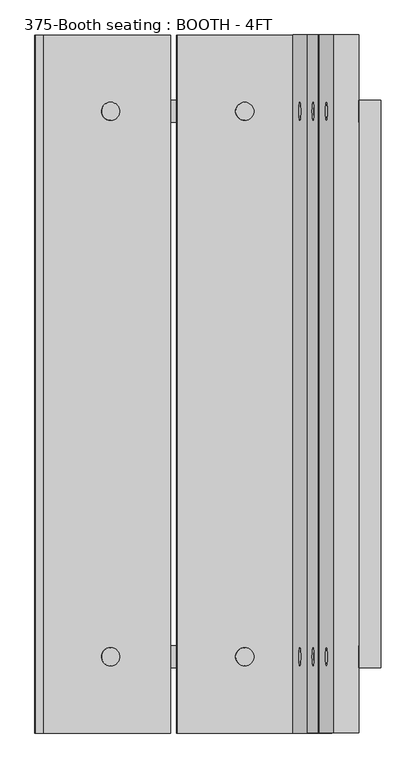
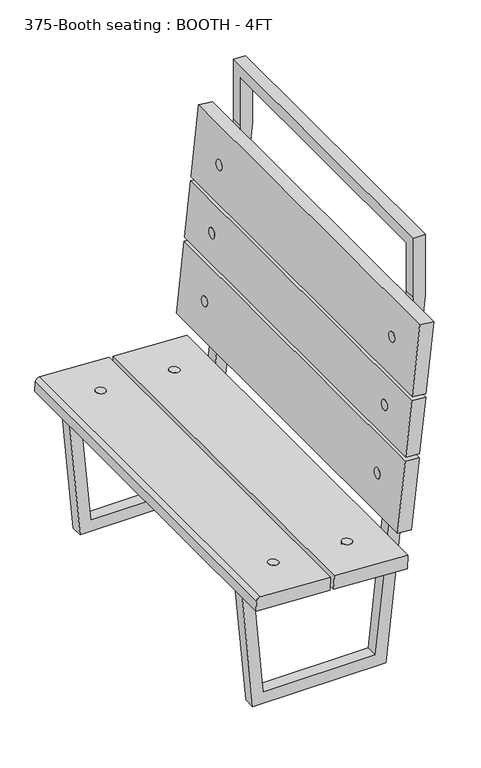
"""IFC4 building model written with IfcOpenShell, lengths in millimetres: furniture geometry, 375-Booth seating : BOOTH - 4FT."""

from ifc_helpers import new_model, si_unit, point, frame, frame_2d, origin, place, context, project, spatial, polyline, circle_curve, trimmed, segment, composite_curve, outline, extrude, faceted_brep, source, transform, mapped, element, save


def furniture_375_booth_seating_booth_4ft_3e2dd1b1(model_context):
    return source(origin(), model_context, "Body", "SolidModel", [
        extrude(outline(composite_curve([segment(trimmed(circle_curve(frame_2d((0.0, 15.875)), 15.875), [point((0.0, 31.75))], [point((0.0, 0.0))], False, "CARTESIAN"), True, "CONTINUOUS"), segment(trimmed(circle_curve(frame_2d((0.0, 15.875)), 15.875), [point((0.0, 0.0))], [point((0.0, 31.75))], False, "CARTESIAN"), True, "CONTINUOUS")], self_intersect=False)), frame((476.8022404, -460.375, 403.0070028), z_axis=(0.052335956242943765, 0.0, 0.9986295347545739), x_axis=(-0.9986295347545739, 0.0, 0.052335956242943765)), (0.0, 0.0, 1.0), 44.45),
        extrude(outline(composite_curve([segment(trimmed(circle_curve(frame_2d((-234.95, 15.875)), 15.875), [point((-234.95, 31.75))], [point((-234.95, 0.0))], False, "CARTESIAN"), True, "CONTINUOUS"), segment(trimmed(circle_curve(frame_2d((-234.95, 15.875)), 15.875), [point((-234.95, 0.0))], [point((-234.95, 31.75))], False, "CARTESIAN"), True, "CONTINUOUS")], self_intersect=False)), frame((476.8022404, -460.375, 403.0070028), z_axis=(0.052335956242943765, 0.0, 0.9986295347545739), x_axis=(-0.9986295347545739, 0.0, 0.052335956242943765)), (0.0, 0.0, 1.0), 44.45),
        extrude(outline(composite_curve([segment(trimmed(circle_curve(frame_2d((0.0, -936.625)), 15.875), [point((0.0, -920.75))], [point((0.0, -952.5))], False, "CARTESIAN"), True, "CONTINUOUS"), segment(trimmed(circle_curve(frame_2d((0.0, -936.625)), 15.875), [point((0.0, -952.5))], [point((0.0, -920.75))], False, "CARTESIAN"), True, "CONTINUOUS")], self_intersect=False)), frame((476.8022404, -460.375, 403.0070028), z_axis=(0.052335956242943765, 0.0, 0.9986295347545739), x_axis=(-0.9986295347545739, 0.0, 0.052335956242943765)), (0.0, 0.0, 1.0), 44.45),
        extrude(outline(composite_curve([segment(trimmed(circle_curve(frame_2d((-234.95, -936.625)), 15.875), [point((-234.95, -920.75))], [point((-234.95, -952.5))], False, "CARTESIAN"), True, "CONTINUOUS"), segment(trimmed(circle_curve(frame_2d((-234.95, -936.625)), 15.875), [point((-234.95, -952.5))], [point((-234.95, -920.75))], False, "CARTESIAN"), True, "CONTINUOUS")], self_intersect=False)), frame((476.8022404, -460.375, 403.0070028), z_axis=(0.052335956242943765, 0.0, 0.9986295347545739), x_axis=(-0.9986295347545739, 0.0, 0.052335956242943765)), (0.0, 0.0, 1.0), 44.45),
        extrude(outline(composite_curve([segment(trimmed(circle_curve(frame_2d((0.0, 15.875)), 15.875), [point((0.0, 31.75))], [point((0.0, 0.0))], False, "CARTESIAN"), True, "CONTINUOUS"), segment(trimmed(circle_curve(frame_2d((0.0, 15.875)), 15.875), [point((0.0, 0.0))], [point((0.0, 31.75))], False, "CARTESIAN"), True, "CONTINUOUS")], self_intersect=False)), frame((900.6975371, 492.125, 1069.1522612), z_axis=(-0.9945218953682735, 0.0, 0.10452846326765225), x_axis=(-0.10452846326765225, 0.0, -0.9945218953682735)), (0.0, 0.0, 1.0), 44.45),
        extrude(outline(composite_curve([segment(trimmed(circle_curve(frame_2d((222.2499999, 15.875)), 15.875), [point((222.2499999, 31.75))], [point((222.2499999, 0.0))], False, "CARTESIAN"), True, "CONTINUOUS"), segment(trimmed(circle_curve(frame_2d((222.2499999, 15.875)), 15.875), [point((222.2499999, 0.0))], [point((222.2499999, 31.75))], False, "CARTESIAN"), True, "CONTINUOUS")], self_intersect=False)), frame((900.6975371, 492.125, 1069.1522612), z_axis=(-0.9945218953682735, 0.0, 0.10452846326765225), x_axis=(-0.10452846326765225, 0.0, -0.9945218953682735)), (0.0, 0.0, 1.0), 44.45),
        extrude(outline(composite_curve([segment(trimmed(circle_curve(frame_2d((444.5, 15.875)), 15.875), [point((444.5, 31.75))], [point((444.5, 0.0))], False, "CARTESIAN"), True, "CONTINUOUS"), segment(trimmed(circle_curve(frame_2d((444.5, 15.875)), 15.875), [point((444.5, 0.0))], [point((444.5, 31.75))], False, "CARTESIAN"), True, "CONTINUOUS")], self_intersect=False)), frame((900.6975371, 492.125, 1069.1522612), z_axis=(-0.9945218953682735, 0.0, 0.10452846326765225), x_axis=(-0.10452846326765225, 0.0, -0.9945218953682735)), (0.0, 0.0, 1.0), 44.45),
        extrude(outline(composite_curve([segment(trimmed(circle_curve(frame_2d((0.0, 968.375)), 15.875), [point((0.0, 984.25))], [point((0.0, 952.5))], False, "CARTESIAN"), True, "CONTINUOUS"), segment(trimmed(circle_curve(frame_2d((0.0, 968.375)), 15.875), [point((0.0, 952.5))], [point((0.0, 984.25))], False, "CARTESIAN"), True, "CONTINUOUS")], self_intersect=False)), frame((900.6975371, 492.125, 1069.1522612), z_axis=(-0.9945218953682735, 0.0, 0.10452846326765225), x_axis=(-0.10452846326765225, 0.0, -0.9945218953682735)), (0.0, 0.0, 1.0), 44.45),
        extrude(outline(composite_curve([segment(trimmed(circle_curve(frame_2d((222.2499999, 968.375)), 15.875), [point((222.2499999, 984.25))], [point((222.2499999, 952.5))], False, "CARTESIAN"), True, "CONTINUOUS"), segment(trimmed(circle_curve(frame_2d((222.2499999, 968.375)), 15.875), [point((222.2499999, 952.5))], [point((222.2499999, 984.25))], False, "CARTESIAN"), True, "CONTINUOUS")], self_intersect=False)), frame((900.6975371, 492.125, 1069.1522612), z_axis=(-0.9945218953682735, 0.0, 0.10452846326765225), x_axis=(-0.10452846326765225, 0.0, -0.9945218953682735)), (0.0, 0.0, 1.0), 44.45),
        extrude(outline(composite_curve([segment(trimmed(circle_curve(frame_2d((444.5, 968.375)), 15.875), [point((444.5, 984.25))], [point((444.5, 952.5))], False, "CARTESIAN"), True, "CONTINUOUS"), segment(trimmed(circle_curve(frame_2d((444.5, 968.375)), 15.875), [point((444.5, 952.5))], [point((444.5, 984.25))], False, "CARTESIAN"), True, "CONTINUOUS")], self_intersect=False)), frame((900.6975371, 492.125, 1069.1522612), z_axis=(-0.9945218953682735, 0.0, 0.10452846326765225), x_axis=(-0.10452846326765225, 0.0, -0.9945218953682735)), (0.0, 0.0, 1.0), 44.45),
        faceted_brep([(828.7442542, 457.2, 384.5625035), (366.8356381, 457.2, 408.7701083), (402.5983885, 457.2, 0.0), (826.6349718, 457.2, 0.0), (952.1084079, 457.2, 1193.8), (952.1084079, 457.2, 1358.9), (914.0084079, 457.2, 1358.9), (914.0084079, 457.2, 1195.7967364), (437.5106063, 457.2, 38.1), (408.6106083, 457.2, 368.4284885), (824.7562543, 457.2, 346.6192193), (792.3295777, 457.2, 38.1), (828.7442542, 495.3, 384.5625035), (914.0084079, 495.3, 1195.7967364), (914.0084079, 495.3, 1397.0), (952.1084079, 495.3, 1397.0), (952.1084079, 495.3, 1193.8), (826.6349718, 495.3, 0.0), (402.5983885, 495.3, 0.0), (366.8356381, 495.3, 408.7701083), (437.5106063, 495.3, 38.1), (792.3295777, 495.3, 38.1), (824.7562543, 495.3, 346.6192193), (408.6106083, 495.3, 368.4284885), (952.1084079, -457.2, 1358.9), (914.0084079, -457.2, 1358.9), (828.7442542, -495.3, 384.5625035), (366.8356381, -495.3, 408.7701083), (402.5983885, -495.3, 0.0), (826.6349718, -495.3, 0.0), (952.1084079, -495.3, 1193.8), (952.1084079, -495.3, 1397.0), (914.0084079, -495.3, 1397.0), (914.0084079, -495.3, 1195.7967364), (437.5106063, -495.3, 38.1), (408.6106083, -495.3, 368.4284885), (824.7562543, -495.3, 346.6192193), (792.3295777, -495.3, 38.1), (828.7442542, -457.2, 384.5625035), (914.0084079, -457.2, 1195.7967364), (952.1084079, -457.2, 1193.8), (826.6349718, -457.2, 0.0), (402.5983885, -457.2, 0.0), (366.8356381, -457.2, 408.7701083), (437.5106063, -457.2, 38.1), (792.3295777, -457.2, 38.1), (824.7562543, -457.2, 346.6192193), (408.6106083, -457.2, 368.4284885)], [[[0, 1, 2, 3, 4, 5, 6, 7], [8, 9, 10, 11]], [[12, 13, 14, 15, 16, 17, 18, 19], [20, 21, 22, 23]], [[3, 17, 16, 4]], [[7, 13, 12, 0]], [[0, 12, 19, 1]], [[1, 19, 18, 2]], [[2, 18, 17, 3]], [[8, 20, 23, 9]], [[9, 23, 22, 10]], [[10, 22, 21, 11]], [[11, 21, 20, 8]], [[6, 5, 24, 25]], [[26, 27, 28, 29, 30, 31, 32, 33], [34, 35, 36, 37]], [[38, 39, 25, 24, 40, 41, 42, 43], [44, 45, 46, 47]], [[26, 38, 43, 27]], [[27, 43, 42, 28]], [[28, 42, 41, 29]], [[34, 44, 47, 35]], [[35, 47, 46, 36]], [[36, 46, 45, 37]], [[37, 45, 44, 34]], [[29, 41, 40, 30]], [[33, 39, 38, 26]], [[15, 31, 30, 40, 24, 5, 4, 16]], [[14, 32, 31, 15]], [[13, 7, 6, 25, 39, 33, 32, 14]]]),
        extrude(outline(polyline([(0.0, 44.45), (1219.2, 44.45), (1219.2, 0.0), (0.0, 0.0), (0.0, 44.45)])), frame((841.955154, -609.6, 510.2558191), z_axis=(0.10452846326765272, 0.0, 0.9945218953682734), x_axis=(0.0, 1.0, 0.0)), (0.0, 0.0, 1.0), 234.95),
        extrude(outline(polyline([(0.0, 44.45), (1219.2, 44.45), (1219.2, 0.0), (0.0, 0.0), (0.0, 44.45)])), frame((867.8416279, -609.6, 756.5491664), z_axis=(0.10452846326765385, 0.0, 0.9945218953682733), x_axis=(0.0, 1.0, 0.0)), (0.0, 0.0, 1.0), 184.15),
        extrude(outline(polyline([(0.0, 44.45), (1219.2, 44.45), (1219.2, 0.0), (0.0, 0.0), (0.0, 44.45)])), frame((888.4180559, -609.6, 952.3208015), z_axis=(0.10452846326765004, 0.0, 0.9945218953682737), x_axis=(0.0, 1.0, 0.0)), (0.0, 0.0, 1.0), 234.95),
        extrude(outline(composite_curve([segment(polyline([(441.9125858, 583.7599832), (453.5442521, 361.8145691)]), True, "CONTINUOUS"), segment(trimmed(circle_curve(frame_2d((440.861657, 361.1499024)), 12.7), [point((453.5442521, 361.8145691))], [point((441.5263237, 348.4673073))], False, "CARTESIAN"), True, "CONTINUOUS"), segment(polyline([(441.5263237, 348.4673073), (409.8198359, 346.8056407), (397.4995564, 581.8905778), (441.9125858, 583.7599832)]), True, "CONTINUOUS")], self_intersect=False)), frame((0.0, -609.6, 0.0), z_axis=(0.0, 1.0, 0.0), x_axis=(0.0, 0.0, 1.0)), (0.0, 0.0, 1.0), 1219.2),
        extrude(outline(polyline([(0.0, 234.95), (1219.2, 234.95), (1219.2, 0.0), (0.0, 0.0), (0.0, 234.95)])), frame((828.7442542, -609.6, 384.5625035), z_axis=(0.05233595624294369, 0.0, 0.9986295347545739), x_axis=(0.0, 1.0, 0.0)), (0.0, 0.0, 1.0), 44.45),
    ])


if __name__ == "__main__":
    model = new_model("IFC4")
    model_context = context("Model", 3, world=origin())
    ifc_project = project(units=[si_unit("LENGTHUNIT", "METRE", prefix="MILLI")], contexts=[model_context])
    site = spatial("IfcSite", under=ifc_project)
    building = spatial("IfcBuilding", under=site)
    placement = place(None, origin())
    furniture_375_booth_seating_booth_4ft_shape = furniture_375_booth_seating_booth_4ft_3e2dd1b1(model_context)
    element("IfcFurniture", 1, ObjectType="375-Booth seating : BOOTH - 4FT", at=placement, inside=building, context=model_context, shape_type="MappedRepresentation", body=[
        mapped(furniture_375_booth_seating_booth_4ft_shape, transform((0.0, 0.0, 0.0), x_axis=(1.0, 0.0, 0.0), y_axis=(0.0, 1.0, 0.0), z_axis=(0.0, 0.0, 1.0))),
    ])
    save(model, "model.ifc")

# Revit data of these elements
# Type "375-Booth seating : BOOTH - 4FT"
#   tube dim [instance default] = 0' - 1 1/2"
#   seat angle = 3.00°
#   radius of plug = 0' - 0 5/8"
#   plank width_2 = 0' - 7 1/4"
#   plank width_1 = 0' - 9 1/4"
#   plank depth = 0' - 1 3/4"
#   inset = 0' - 6"
#   gap = 0' - 0 1/2"
#   DEPTH = 4' - 0"
#   Seating Count = 2
#   middle support visibility = no
#   Right Bench Visible [instance default] = yes
#   Left Bench Visible [instance default] = yes
#   Material_1 = WOOD-OAKFIRE
#   Material 2 = 1 1/2" SQUARE TUBE STEEL\n- WELDED MITER JOINTS GROUND SMOOTH\n- CLEAR COAT
#   Assembly Code = ""
# Element 1 (IfcFurniture, "375-Booth seating : BOOTH - 4FT")
#   Materials on its faces: "1 1/2\" SQUARE TUBE STEEL\n- WELDED MITER JOINTS GROUND SMOOTH\n- CLEAR COAT", "WOOD-OAKFIRE", "1 1/4\" WOOD PLUG\n(SLIGHTLY DARKER OR STAINED WOOD) - GAL. HEX HEAD THRU BOLT"
# Materials
#   "WOOD-OAKFIRE": class "Wood", colour RGB 198 202 183, transparency 0, Description = "Generic wood", Cost = 0
#   "1 1/2\" SQUARE TUBE STEEL\n- WELDED MITER JOINTS GROUND SMOOTH\n- CLEAR COAT": class "Metal", colour RGB 147 147 147, transparency 0, Cost = 0
#   "1 1/4\" WOOD PLUG\n(SLIGHTLY DARKER OR STAINED WOOD) - GAL. HEX HEAD THRU BOLT": class "Generic", colour RGB 192 192 192, transparency 0, Cost = 0
